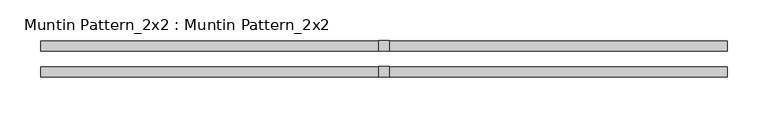
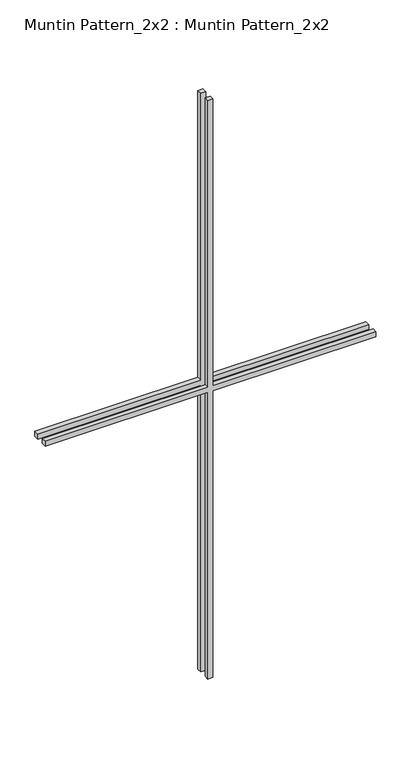
"""IFC4 building model written with IfcOpenShell, lengths in millimetres: proxy geometry, Muntin Pattern_2x2 : Muntin Pattern_2x2."""

import ifcopenshell
import ifcopenshell.guid

model = None  # the IFC model being written
_history = None  # IfcOwnerHistory: only IFC2X3 demands one
_inside = {}  # id of a spatial element -> (the spatial element, [elements in it])
_under = {}  # id of a project, library or spatial element -> (it, [spatial elements below it])
_declared = {}  # id of a project -> (the project, [libraries it declares])
_typed = {}  # id of a type object -> (the type object, [elements of that type])
_made_of = {}  # id of a material, layer set ... -> (it, [elements and type objects made of it])


def new_model(schema):
    """Start an empty IFC model of exactly this schema.

    Asked for "IFC4X3", IfcOpenShell would pick the latest addendum, in which some entities
    have other attributes; the version numbers below select the first issue.
    IFC2X3 requires an IfcOwnerHistory on every rooted entity: one is made here for all.
    """
    global model, _history
    if schema == "IFC4X3":
        model = ifcopenshell.file(schema_version=(4, 3, 0, 0))
    else:
        model = ifcopenshell.file(schema=schema)
    _inside.clear()
    _under.clear()
    _declared.clear()
    _typed.clear()
    _made_of.clear()
    _history = None
    if model.schema == "IFC2X3":
        org = make("IfcOrganization", Name="unknown")
        user = make(
            "IfcPersonAndOrganization",
            ThePerson=make("IfcPerson", FamilyName="unknown"),
            TheOrganization=org,
        )
        app = make(
            "IfcApplication",
            ApplicationDeveloper=org,
            Version="unknown",
            ApplicationFullName="unknown",
            ApplicationIdentifier="unknown",
        )
        _history = make(
            "IfcOwnerHistory",
            OwningUser=user,
            OwningApplication=app,
            ChangeAction="ADDED",
            CreationDate=0,
        )
    return model


def make(cls, **values):
    """One entity of the class cls with the attributes given. An attribute that is None is left unset."""
    return model.create_entity(
        cls, **{name: value for name, value in values.items() if value is not None}
    )


def rooted(cls, **values):
    """An entity with a GlobalId (a new one), such as an element, a storey or a relation."""
    return make(cls, GlobalId=ifcopenshell.guid.new(), OwnerHistory=_history, **values)


def si_unit(unit_type, name, prefix=None):
    """IfcSIUnit, for example si_unit("LENGTHUNIT", "METRE", prefix="MILLI")."""
    return make("IfcSIUnit", UnitType=unit_type, Prefix=prefix, Name=name)


def assignment(units):
    """IfcUnitAssignment: the units of a project."""
    return None if units is None else make("IfcUnitAssignment", Units=units)


def point(xyz):
    """IfcCartesianPoint."""
    return None if xyz is None else make("IfcCartesianPoint", Coordinates=xyz)


def direction(xyz):
    """IfcDirection."""
    return None if xyz is None else make("IfcDirection", DirectionRatios=xyz)


def frame(location, z_axis=None, x_axis=None):
    """IfcAxis2Placement3D, a coordinate frame: its origin and axes. An axis left out is left unset."""
    return make(
        "IfcAxis2Placement3D",
        Location=point(location),
        Axis=direction(z_axis),
        RefDirection=direction(x_axis),
    )


def origin():
    """The frame at (0, 0, 0) with its axes left unset."""
    return frame((0.0, 0.0, 0.0))


def place(relative_to, where):
    """IfcLocalPlacement: puts the frame where relative to a parent placement (None: the world)."""
    return make(
        "IfcLocalPlacement", PlacementRelTo=relative_to, RelativePlacement=where
    )


def context(
    kind, dimensions, precision=None, world=None, true_north=None, identifier=None
):
    """IfcGeometricRepresentationContext, for example the 3D "Model" context."""
    return make(
        "IfcGeometricRepresentationContext",
        ContextIdentifier=identifier,
        ContextType=kind,
        CoordinateSpaceDimension=dimensions,
        Precision=precision,
        WorldCoordinateSystem=world,
        TrueNorth=true_north,
    )


def project(units=None, contexts=None):
    """IfcProject with its units and contexts."""
    return rooted(
        "IfcProject",
        Name="project",
        RepresentationContexts=contexts,
        UnitsInContext=assignment(units),
    )


def spatial(cls, under=None, at=None, **own):
    """A site, building, storey or space (cls), placed at a placement, below another one or the project."""
    s = rooted(cls, ObjectPlacement=at, **own)
    if under is not None:
        _under.setdefault(under.id(), (under, []))[1].append(s)
    return s


def polyline(points):
    """IfcPolyline through the points."""
    return make("IfcPolyline", Points=[point(p) for p in points])


def outline(outer, holes=None, kind="AREA"):
    """IfcArbitraryClosedProfileDef: a profile drawn as a closed curve; with holes, ...WithVoids."""
    if holes is None:
        return make("IfcArbitraryClosedProfileDef", ProfileType=kind, OuterCurve=outer)
    return make(
        "IfcArbitraryProfileDefWithVoids",
        ProfileType=kind,
        OuterCurve=outer,
        InnerCurves=holes,
    )


def extrude(swept, where, along, depth):
    """IfcExtrudedAreaSolid: the profile swept, set in the frame where, extruded along a direction by depth."""
    return make(
        "IfcExtrudedAreaSolid",
        SweptArea=swept,
        Position=where,
        ExtrudedDirection=direction(along),
        Depth=depth,
    )


def shape(context_of_items, identifier, shape_type, items):
    """IfcShapeRepresentation: the items that make up one representation, for example the "Body"."""
    return make(
        "IfcShapeRepresentation",
        ContextOfItems=context_of_items,
        RepresentationIdentifier=identifier,
        RepresentationType=shape_type,
        Items=items,
    )


def source(mapping_origin, context_of_items, identifier, shape_type, items):
    """IfcRepresentationMap: a shape defined once, which mapped items show again and again."""
    return make(
        "IfcRepresentationMap",
        MappingOrigin=mapping_origin,
        MappedRepresentation=shape(context_of_items, identifier, shape_type, items),
    )


def transform(
    local_origin,
    x_axis=None,
    y_axis=None,
    z_axis=None,
    scale=None,
    scale2=None,
    scale3=None,
    uniform=True,
):
    """IfcCartesianTransformationOperator3D, or its non-uniform kind. x_axis, y_axis, z_axis: its Axis1, 2, 3."""
    if uniform:
        return make(
            "IfcCartesianTransformationOperator3D",
            Axis1=direction(x_axis),
            Axis2=direction(y_axis),
            LocalOrigin=point(local_origin),
            Scale=scale,
            Axis3=direction(z_axis),
        )
    return make(
        "IfcCartesianTransformationOperator3DnonUniform",
        Axis1=direction(x_axis),
        Axis2=direction(y_axis),
        LocalOrigin=point(local_origin),
        Scale=scale,
        Axis3=direction(z_axis),
        Scale2=scale2,
        Scale3=scale3,
    )


def mapped(mapping_source, mapping_target):
    """IfcMappedItem: shows the shape of a source again, moved by a transform."""
    return make(
        "IfcMappedItem", MappingSource=mapping_source, MappingTarget=mapping_target
    )


def made_of(thing, what):
    """Note that an element or type object is made of a material, layer set ...; save() writes the relation."""
    if what is not None:
        _made_of.setdefault(what.id(), (what, []))[1].append(thing)
    return thing


def element(
    cls,
    number,
    at=None,
    inside=None,
    cuts=None,
    type_object=None,
    material=None,
    context=None,
    identifier="Body",
    shape_type=None,
    held_by="IfcProductDefinitionShape",
    body=None,
    shapes=None,
    **own,
):
    """One element of the class cls, such as IfcWall. Its Tag is "e" and its number.

    at: its placement. inside: the storey or other place that contains it. cuts: it is an
    opening in that element (IfcRelVoidsElement). A single representation is given by context,
    identifier, shape_type and body (its items); several are given by shapes. held_by: the class
    of the entity that holds the representations. save() writes the other relations.
    """
    e = rooted(cls, Tag="e%d" % number, ObjectPlacement=at, **own)
    if body is not None:
        shapes = [shape(context, identifier, shape_type, body)]
    if shapes is not None:
        e.Representation = make(held_by, Representations=shapes)
    if inside is not None:
        _inside.setdefault(inside.id(), (inside, []))[1].append(e)
    if cuts is not None:
        rooted(
            "IfcRelVoidsElement", RelatingBuildingElement=cuts, RelatedOpeningElement=e
        )
    if type_object is not None:
        _typed.setdefault(type_object.id(), (type_object, []))[1].append(e)
    return made_of(e, material)


def aggregate(whole, parts):
    """IfcRelAggregates: a whole, such as a stair, and the parts it consists of."""
    return rooted("IfcRelAggregates", RelatingObject=whole, RelatedObjects=parts)


def save(model, path):
    """Write the relations noted so far, then the file.

    IfcRelAggregates (storeys below a building ...), IfcRelContainedInSpatialStructure (elements
    in a storey), IfcRelDefinesByType, IfcRelAssociatesMaterial and IfcRelDeclares: one each for
    every whole, place, type object, material and project.
    """
    for whole, parts in _under.values():
        aggregate(whole, parts)
    for where, things in _inside.values():
        rooted(
            "IfcRelContainedInSpatialStructure",
            RelatedElements=things,
            RelatingStructure=where,
        )
    for kind, things in _typed.values():
        rooted("IfcRelDefinesByType", RelatedObjects=things, RelatingType=kind)
    for what, things in _made_of.values():
        rooted("IfcRelAssociatesMaterial", RelatedObjects=things, RelatingMaterial=what)
    for by, libraries in _declared.values():
        rooted("IfcRelDeclares", RelatingContext=by, RelatedDefinitions=libraries)
    model.write(path)


def muntin_pattern_2x2_muntin_pattern_2x2_e27c8d0d(model_context):
    return source(origin(), model_context, "Body", "SweptSolid", [
        extrude(outline(polyline([(781.05, -6.35), (781.05, -419.1), (768.35, -419.1), (768.35, -6.35), (0.0, -6.35), (0.0, 6.35), (768.35, 6.35), (768.35, 419.1), (781.05, 419.1), (781.05, 6.35), (1549.4, 6.35), (1549.4, -6.35), (781.05, -6.35)])), frame((0.0, -22.225, 0.0), z_axis=(0.0, 1.0, 0.0), x_axis=(0.0, 0.0, 1.0)), (0.0, 0.0, 1.0), 12.7),
        extrude(outline(polyline([(781.05, -6.35), (781.05, -419.1), (768.35, -419.1), (768.35, -6.35), (0.0, -6.35), (0.0, 6.35), (768.35, 6.35), (768.35, 419.1), (781.05, 419.1), (781.05, 6.35), (1549.4, 6.35), (1549.4, -6.35), (781.05, -6.35)])), frame((0.0, 9.525, 0.0), z_axis=(0.0, 1.0, 0.0), x_axis=(0.0, 0.0, 1.0)), (0.0, 0.0, 1.0), 12.7),
    ])


if __name__ == "__main__":
    model = new_model("IFC4")
    model_context = context("Model", 3, world=origin())
    ifc_project = project(units=[si_unit("LENGTHUNIT", "METRE", prefix="MILLI")], contexts=[model_context])
    site = spatial("IfcSite", under=ifc_project)
    building = spatial("IfcBuilding", under=site)
    placement = place(None, origin())
    muntin_pattern_2x2_muntin_pattern_2x2_shape = muntin_pattern_2x2_muntin_pattern_2x2_e27c8d0d(model_context)
    element("IfcBuildingElementProxy", 1, Name="Muntin Pattern_2x2 : Muntin Pattern_2x2", ObjectType="Muntin Pattern_2x2 : Muntin Pattern_2x2", at=placement, inside=building, context=model_context, shape_type="MappedRepresentation", body=[
        mapped(muntin_pattern_2x2_muntin_pattern_2x2_shape, transform((0.0, 0.0, 0.0), x_axis=(1.0, 0.0, 0.0), y_axis=(0.0, 1.0, 0.0), z_axis=(0.0, 0.0, 1.0))),
    ])
    save(model, "model.ifc")

# Revit data of these elements
# Type "Muntin Pattern_2x2 : Muntin Pattern_2x2"
#   Width [instance default] = 4' - 0"
#   Thickness = 0' - 0 1/2"
#   Height [instance default] = 4' - 0"
#   Distance = 0' - 0 3/4"
#   Interior Material [instance default] = none
#   Exterior Material [instance default] = none
#   Default Elevation = 0
# Element 1 (IfcBuildingElementProxy, "Muntin Pattern_2x2 : Muntin Pattern_2x2")
#   Width = 2' - 9"
#   Height = 5' - 1"
#   Interior Material = Wood - Stained
#   Exterior Material = Clad - White
#   Materials on its faces: "Clad - White", "Wood - Stained"
# Materials
#   "Clad - White": class "Wood", colour RGB 242 242 238, transparency 0, Cost = 0
#   "Wood - Stained": class "Wood", colour RGB 224 178 126, transparency 0, Cost = 0
